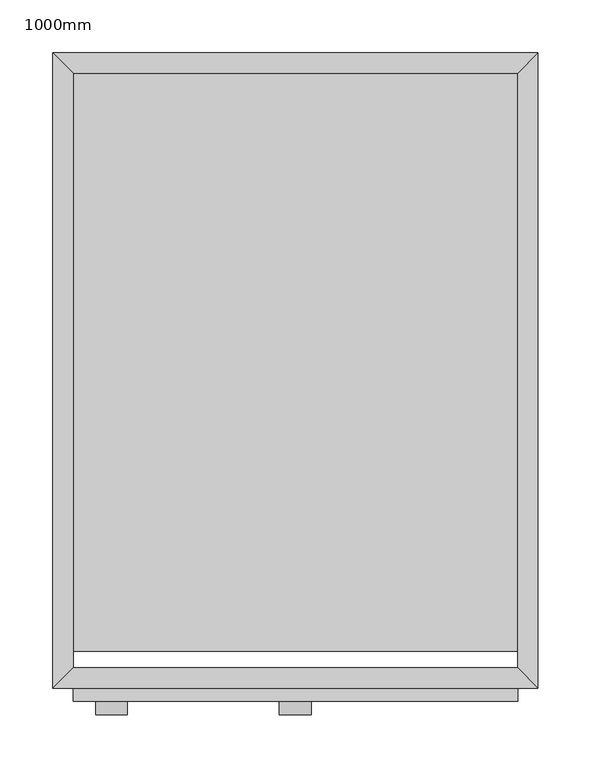
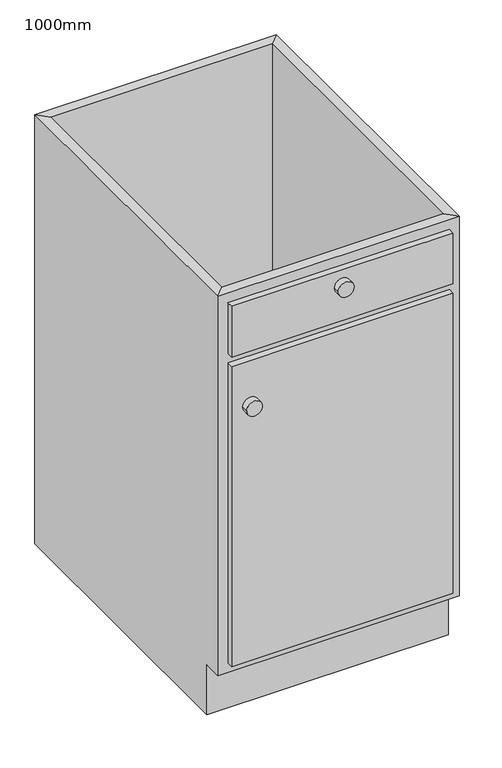
"""IFC4 building model written with IfcOpenShell, lengths in millimetres: furniture geometry, M_Base Cabinet-single &  Drawer-ROUND : 1000mm."""

from ifc_helpers import new_model, si_unit, point, frame, frame_2d, origin, place, context, project, spatial, polyline, circle_curve, trimmed, segment, composite_curve, outline, extrude, faceted_brep, source, transform, mapped, element, save


def furniture_1000mm_0fea18c1(model_context):
    return source(origin(), model_context, "Body", "SolidModel", [
        faceted_brep([(507.6877049, -580.95, 860.0), (507.6877049, -580.95, 100.0), (87.7877049, -580.95, 100.0), (87.7877049, -580.95, 860.0), (68.7377049, -600.0, 860.0), (526.7377049, -600.0, 860.0), (68.7377049, -600.0, 100.0), (526.7377049, -600.0, 100.0), (87.7877049, -565.0, 100.0), (87.7877049, -19.05, 100.0), (87.7877049, -19.05, 860.0), (68.7377049, 0.0, 860.0), (68.7377049, 0.0, 0.0), (68.7377049, -565.0, 0.0), (68.7377049, -565.0, 100.0), (507.6877049, -19.05, 100.0), (507.6877049, -19.05, 860.0), (526.7377049, 0.0, 860.0), (526.7377049, 0.0, 0.0), (507.6877049, -565.0, 100.0), (526.7377049, -565.0, 100.0), (526.7377049, -565.0, 0.0)], [[[0, 1, 2, 3]], [[0, 3, 4, 5]], [[5, 4, 6, 7]], [[2, 1, 7, 6]], [[3, 2, 8, 9, 10]], [[4, 3, 10, 11]], [[6, 4, 11, 12, 13, 14]], [[2, 6, 14, 8]], [[10, 9, 15, 16]], [[11, 10, 16, 17]], [[11, 17, 18, 12]], [[1, 0, 16, 15, 19]], [[0, 5, 17, 16]], [[5, 7, 20, 21, 18, 17]], [[7, 1, 19, 20]], [[8, 19, 15, 9]], [[18, 21, 13, 12]], [[13, 21, 20, 19, 8, 14]]]),
        extrude(outline(composite_curve([segment(trimmed(circle_curve(frame_2d((809.2, 297.7377049)), 15.0), [point((809.2, 282.7377049))], [point((809.2, 312.7377049))], False, "CARTESIAN"), True, "CONTINUOUS"), segment(trimmed(circle_curve(frame_2d((809.2, 297.7377049)), 15.0), [point((809.2, 312.7377049))], [point((809.2, 282.7377049))], False, "CARTESIAN"), True, "CONTINUOUS")], self_intersect=False)), frame((0.0, -625.4, 0.0), z_axis=(0.0, 1.0, 0.0), x_axis=(0.0, 0.0, 1.0)), (0.0, 0.0, 1.0), 12.7),
        extrude(outline(composite_curve([segment(trimmed(circle_curve(frame_2d((631.4, 124.0127049)), 15.0), [point((631.4, 109.0127049))], [point((631.4, 139.0127049))], False, "CARTESIAN"), True, "CONTINUOUS"), segment(trimmed(circle_curve(frame_2d((631.4, 124.0127049)), 15.0), [point((631.4, 139.0127049))], [point((631.4, 109.0127049))], False, "CARTESIAN"), True, "CONTINUOUS")], self_intersect=False)), frame((0.0, -625.4, 0.0), z_axis=(0.0, 1.0, 0.0), x_axis=(0.0, 0.0, 1.0)), (0.0, 0.0, 1.0), 12.7),
        extrude(outline(polyline([(507.6877049, -612.7), (87.7877049, -612.7), (87.7877049, -600.0), (507.6877049, -600.0), (507.6877049, -612.7)])), frame((0.0, 0.0, 739.35), z_axis=(0.0, 0.0, 1.0), x_axis=(1.0, 0.0, 0.0)), (0.0, 0.0, 1.0), 101.6),
        extrude(outline(polyline([(507.6877049, -612.7), (87.7877049, -612.7), (87.7877049, -600.0), (507.6877049, -600.0), (507.6877049, -612.7)])), frame((0.0, 0.0, 119.05), z_axis=(0.0, 0.0, 1.0), x_axis=(1.0, 0.0, 0.0)), (0.0, 0.0, 1.0), 601.25),
    ])


if __name__ == "__main__":
    model = new_model("IFC4")
    model_context = context("Model", 3, world=origin())
    ifc_project = project(units=[si_unit("LENGTHUNIT", "METRE", prefix="MILLI")], contexts=[model_context])
    site = spatial("IfcSite", under=ifc_project)
    building = spatial("IfcBuilding", under=site)
    placement = place(None, origin())
    furniture_1000mm_shape = furniture_1000mm_0fea18c1(model_context)
    element("IfcFurniture", 1, ObjectType="M_Base Cabinet-single &  Drawer-ROUND : 1000mm", at=placement, inside=building, context=model_context, shape_type="MappedRepresentation", body=[
        mapped(furniture_1000mm_shape, transform((0.0, 0.0, 0.0), x_axis=(1.0, 0.0, 0.0), y_axis=(0.0, 1.0, 0.0), z_axis=(0.0, 0.0, 1.0))),
    ])
    save(model, "model.ifc")

# Revit data of these elements
# Type "M_Base Cabinet-single &  Drawer-ROUND : 1000mm"
#   Depth = 1' - 11.62205"
#   Height = 2' - 9.85827"
#   Plinth Depth = 0' - 1.37795"
#   Plinth Height = 0' - 3.93701"
#   Width = 3' - 4"
#   Cabinet Material = Base cabinet 2120100 Aspekt - 83012120100 - White
#   Door/Drawer Material = Base cabinet 2120100 Aspekt - 83012120100 - White
#   Handle Material = Cabinets - Handles
#   Default Elevation = 0
# Element 1 (IfcFurniture, "M_Base Cabinet-single &  Drawer-ROUND : 1000mm")
#   Materials on its faces: "Base cabinet 2120100 Aspekt - 83012120100 - White", "Cabinets - Handles"
# Materials
#   "Base cabinet 2120100 Aspekt - 83012120100 - White": class "Miscellaneous", colour RGB 255 255 255, transparency 0, Manufacturer = "Marbodal", URL = "http://www.marbodal.se", Cost = 0
#   "Cabinets - Handles": class "Metal", colour RGB 57 57 57, transparency 0
